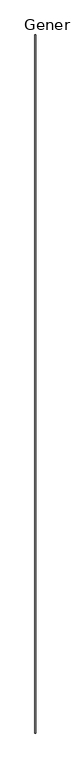
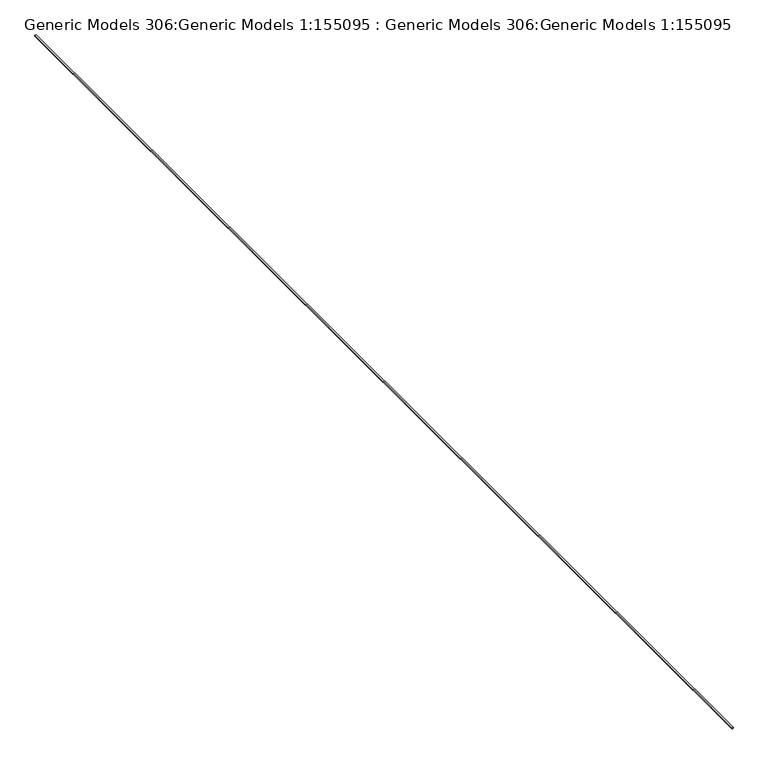
"""IFC4 building model written with IfcOpenShell, lengths in millimetres: proxy geometry, Generic Models 306:Generic Models 1:155095 : Generic Models 306:Generic Models 1:155095."""

from ifc_helpers import new_model, si_unit, point, frame, frame_2d, origin, place, context, project, spatial, polyline, circle_curve, trimmed, segment, composite_curve, outline, extrude, source, transform, mapped, element, save


def generic_models_306_generic_models_1_155095_generic_models_1d5753ed(model_context):
    return source(origin(), model_context, "Body", "SweptSolid", [
        extrude(outline(composite_curve([segment(trimmed(circle_curve(frame_2d((82.029481, 7127.753213)), 8.620055), [point((76.2, 7134.103213))], [point((76.2, 7121.403213))], True, "CARTESIAN"), True, "CONTINUOUS"), segment(polyline([(76.2, 7121.403213), (66.675, 7121.403213)]), True, "CONTINUOUS"), segment(trimmed(circle_curve(frame_2d((72.504481, 7127.753213)), 8.620055), [point((66.675, 7121.403213))], [point((66.675, 7134.103213))], False, "CARTESIAN"), True, "CONTINUOUS"), segment(polyline([(66.675, 7134.103213), (76.2, 7134.103213)]), True, "CONTINUOUS")], self_intersect=False)), frame((0.0, 8191.2927644, 0.0), z_axis=(0.0, 1.0, 0.0), x_axis=(0.0, 0.0, 1.0)), (0.0, 0.0, 1.0), 12344.4),
    ])


if __name__ == "__main__":
    model = new_model("IFC4")
    model_context = context("Model", 3, world=origin())
    ifc_project = project(units=[si_unit("LENGTHUNIT", "METRE", prefix="MILLI")], contexts=[model_context])
    site = spatial("IfcSite", under=ifc_project)
    building = spatial("IfcBuilding", under=site)
    placement = place(None, origin())
    generic_models_306_generic_models_1_155095_generic_models_shape = generic_models_306_generic_models_1_155095_generic_models_1d5753ed(model_context)
    element("IfcBuildingElementProxy", 1, Name="Generic Models 306:Generic Models 1:155095 : Generic Models 306:Generic Models 1:155095", ObjectType="Generic Models 306:Generic Models 1:155095 : Generic Models 306:Generic Models 1:155095", at=placement, inside=building, context=model_context, shape_type="MappedRepresentation", body=[
        mapped(generic_models_306_generic_models_1_155095_generic_models_shape, transform((0.0, 0.0, 0.0), x_axis=(1.0, 0.0, 0.0), y_axis=(0.0, 1.0, 0.0), z_axis=(0.0, 0.0, 1.0))),
    ])
    save(model, "model.ifc")

# Revit data of these elements
# Type "Generic Models 306:Generic Models 1:155095 : Generic Models 306:Generic Models 1:155095"
#   NameOverride = "Generic Models 306:Generic Models 1:155095"
#   ObjectTypeOverride = "Generic Models 306:Generic Models 1"
#   Reference = "Generic Models 1"
#   Category = "Generic Models"
#   Tag = "155095"
# Element 1 (IfcBuildingElementProxy, "Generic Models 306:Generic Models 1:155095 : Generic Models 306:Generic Models 1:155095")
#   Materials on its faces: "_SEALANT JOINT 27113"
# Materials
#   "_SEALANT JOINT 27113": class "Unassigned", colour RGB 190 220 196, transparency 0
